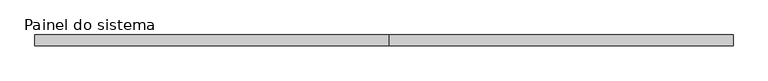
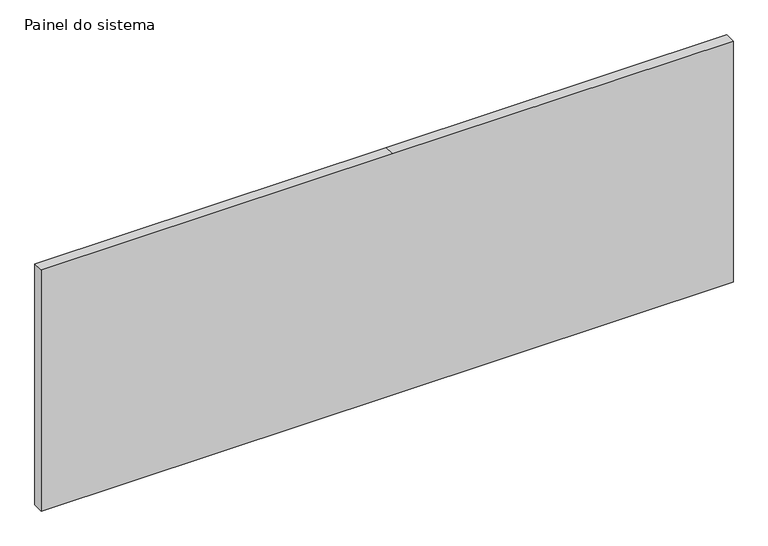
"""IFC4 building model written with IfcOpenShell, lengths in millimetres: plate geometry, Painel do sistema : Envidraçado."""

from ifc_helpers import new_model, si_unit, frame, origin, place, context, project, spatial, polyline, outline, extrude, source, transform, mapped, element, save


def painel_do_sistema_b00e55f7(model_context):
    return source(origin(), model_context, "Body", "SweptSolid", [
        extrude(outline(polyline([(0.0, -800.0500001), (0.0, 12.4999998), (0.0, 800.0500001), (590.0, 800.0500001), (590.0, 12.4999998), (590.0, -800.0500001), (0.0, -800.0500001)])), frame((0.0, -49.5, 0.0), z_axis=(0.0, 1.0, 0.0), x_axis=(0.0, 0.0, 1.0)), (0.0, 0.0, 1.0), 25.0),
    ])


if __name__ == "__main__":
    model = new_model("IFC4")
    model_context = context("Model", 3, world=origin())
    ifc_project = project(units=[si_unit("LENGTHUNIT", "METRE", prefix="MILLI")], contexts=[model_context])
    site = spatial("IfcSite", under=ifc_project)
    building = spatial("IfcBuilding", under=site)
    placement = place(None, origin())
    painel_do_sistema_shape = painel_do_sistema_b00e55f7(model_context)
    element("IfcPlate", 1, ObjectType="Painel do sistema : Envidraçado", at=placement, inside=building, context=model_context, shape_type="MappedRepresentation", body=[
        mapped(painel_do_sistema_shape, transform((0.0, 0.0, 0.0), x_axis=(1.0, 0.0, 0.0), y_axis=(0.0, 1.0, 0.0), z_axis=(0.0, 0.0, 1.0))),
    ])
    save(model, "model.ifc")

# Revit data of these elements
# Type "Painel do sistema : Envidraçado"
#   Construction Type Id = "GSP4R"
#   Analytic Construction = "Vidraça única Pilkington 1/8 pol"
#   Visual Light Transmittance = 0.9
#   Solar Heat Gain Coefficient = 0.86
#   Heat Transfer Coefficient (U) = 6.7069 W/(m²·K)
# Element 1 (IfcPlate, "Painel do sistema : Envidraçado")
#   Materials on its faces: ".VIDRO GENÉRICO"
# Materials
#   ".VIDRO GENÉRICO": class ".CC_VIDRO", colour RGB 0 128 192, transparency 0.9, Description = "Vidro comum", Cost = 0
